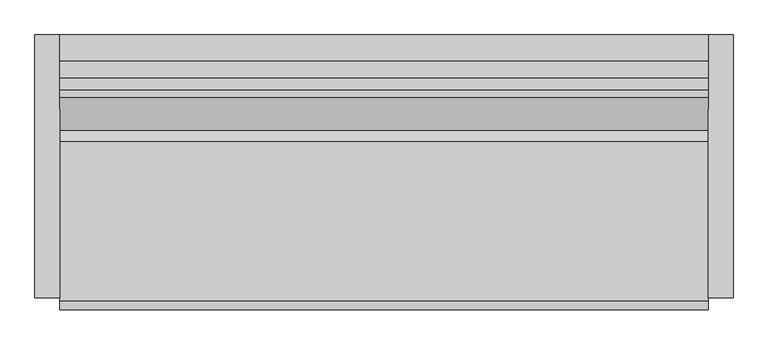
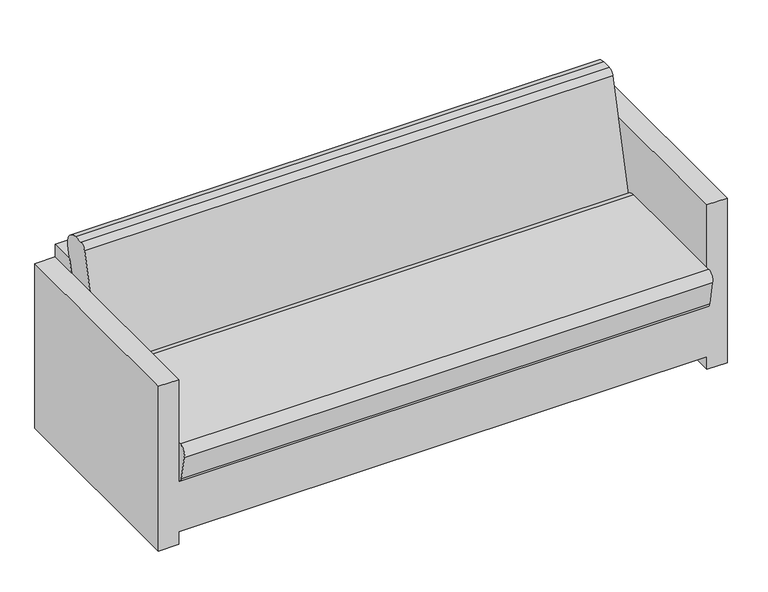
"""IFC4 building model written with IfcOpenShell, lengths in millimetres: furniture geometry, Sofa, 3-Seat-NON-COLLECTUS : -."""

from ifc_helpers import new_model, si_unit, point, frame, frame_2d, origin, place, context, project, spatial, polyline, circle_curve, trimmed, segment, composite_curve, outline, extrude, faceted_brep, source, transform, mapped, element, save


def furniture_0bb38a02(model_context):
    return source(origin(), model_context, "Body", "SolidModel", [
        faceted_brep([(76.2, 35.4707031, 0.0), (76.2, 838.2, 0.0), (76.2, 838.2, 50.0), (76.2, 35.4707031, 50.0), (76.2, 731.5897206, 652.8), (76.2, 35.4707031, 652.8), (76.2, 35.4707031, 250.0), (76.2, 631.7814304, 250.0), (0.0, 838.2, 0.0), (0.0, 35.4707031, 0.0), (0.0, 35.4707031, 652.8), (0.0, 838.2, 652.8), (76.2, 838.2, 652.8), (76.2, 838.2, 702.8), (2057.4, 838.2, 702.8), (2057.4, 838.2, 652.8), (2133.6, 838.2, 652.8), (2133.6, 838.2, 0.0), (2057.4, 838.2, 0.0), (2057.4, 838.2, 50.0), (2057.4, 35.4707031, 50.0), (2057.4, 35.4707031, 0.0), (2133.6, 35.4707031, 0.0), (2133.6, 35.4707031, 652.8), (2057.4, 35.4707031, 652.8), (2057.4, 35.4707031, 250.0), (2057.4, 743.9790317, 702.8), (2057.4, 731.5897206, 652.8), (76.2, 743.9790317, 702.8), (2057.4, 631.7814304, 250.0)], [[[0, 1, 2, 3]], [[4, 5, 6, 7]], [[8, 9, 10, 11]], [[8, 11, 12, 13, 14, 15, 16, 17, 18, 19, 2, 1]], [[11, 10, 5, 4, 12]], [[10, 9, 0, 3, 20, 21, 22, 23, 24, 25, 6, 5]], [[1, 0, 9, 8]], [[14, 26, 27, 15]], [[28, 13, 12, 4]], [[29, 7, 6, 25]], [[20, 3, 2, 19]], [[26, 14, 13, 28]], [[7, 29, 27, 26, 28, 4]], [[17, 16, 23, 22]], [[25, 24, 27, 29]], [[18, 21, 20, 19]], [[23, 16, 15, 27, 24]], [[17, 22, 21, 18]]]),
        extrude(outline(composite_curve([segment(polyline([(755.6205127, 749.7819547), (631.7814304, 250.0), (42.6318449, 250.0)]), True, "CONTINUOUS"), segment(trimmed(circle_curve(frame_2d((42.6318449, 275.0)), 25.0), [point((42.6318449, 250.0))], [point((18.011651, 270.6587956))], False, "CARTESIAN"), True, "CONTINUOUS"), segment(polyline([(18.011651, 270.6587956), (-0.1218553, 365.4877295)]), True, "CONTINUOUS"), segment(trimmed(circle_curve(frame_2d((25.8559684, 375.7732675)), 27.9399287), [point((-0.1218553, 365.4877295))], [point((25.8559684, 403.7131962))], False, "CARTESIAN"), True, "CONTINUOUS"), segment(polyline([(25.8559684, 403.7131962), (512.0757528, 403.7131962)]), True, "CONTINUOUS"), segment(trimmed(circle_curve(frame_2d((512.0757528, 356.7601754)), 46.9530208), [point((512.0757528, 403.7131962))], [point((546.2661504, 388.9409597))], False, "CARTESIAN"), True, "CONTINUOUS"), segment(polyline([(546.2661504, 388.9409597), (646.5125422, 793.5090227)]), True, "CONTINUOUS"), segment(trimmed(circle_curve(frame_2d((671.1669504, 787.4)), 25.4), [point((646.5125422, 793.5090227))], [point((671.1669504, 812.8))], False, "CARTESIAN"), True, "CONTINUOUS"), segment(polyline([(671.1669504, 812.8), (706.3116964, 812.8)]), True, "CONTINUOUS"), segment(trimmed(circle_curve(frame_2d((706.3116964, 762.0)), 50.8), [point((706.3116964, 812.8))], [point((755.6205127, 749.7819547))], False, "CARTESIAN"), True, "CONTINUOUS")], self_intersect=False)), frame((76.2, 0.0, 0.0), z_axis=(1.0, 0.0, 0.0), x_axis=(0.0, 1.0, 0.0)), (0.0, 0.0, 1.0), 1981.2),
    ])


if __name__ == "__main__":
    model = new_model("IFC4")
    model_context = context("Model", 3, world=origin())
    ifc_project = project(units=[si_unit("LENGTHUNIT", "METRE", prefix="MILLI")], contexts=[model_context])
    site = spatial("IfcSite", under=ifc_project)
    building = spatial("IfcBuilding", under=site)
    placement = place(None, origin())
    furniture_shape = furniture_0bb38a02(model_context)
    element("IfcFurniture", 1, ObjectType="Sofa, 3-Seat-NON-COLLECTUS : -", at=placement, inside=building, context=model_context, shape_type="MappedRepresentation", body=[
        mapped(furniture_shape, transform((0.0, 0.0, 0.0), x_axis=(1.0, 0.0, 0.0), y_axis=(0.0, 1.0, 0.0), z_axis=(0.0, 0.0, 1.0))),
    ])
    save(model, "model.ifc")

# Revit data of these elements
# Type "Sofa, 3-Seat-NON-COLLECTUS : -"
#   External ID [instance default] = ""
#   projection = 35.52 mm
#   Width = 2133.6 mm
#   Height = 812.8 mm
#   Depth = 838.2 mm
#   Arm Width = 76.2 mm
#   Frame = White
#   Cushion = White
#   Default Elevation = 0
# Element 1 (IfcFurniture, "Sofa, 3-Seat-NON-COLLECTUS : -")
#   Materials on its faces: "White"
# Materials
#   "White": class "Generic", colour RGB 255 255 255, transparency 0, Cost = 0
